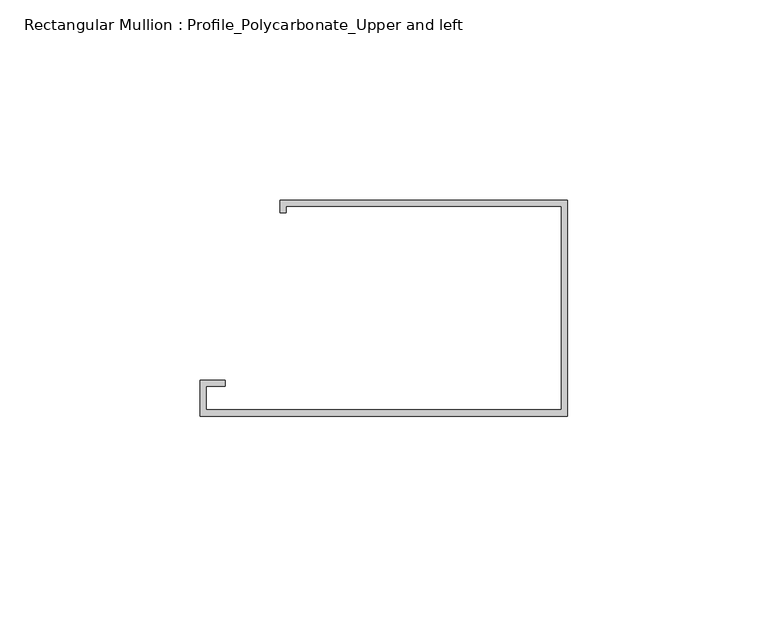
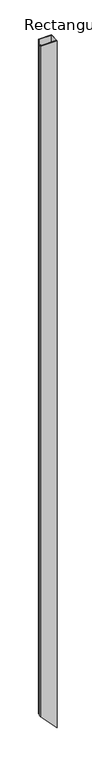
"""IFC4 building model written with IfcOpenShell, lengths in millimetres: member geometry, Rectangular Mullion : Profile_Polycarbonate_Upper and left."""

from ifc_helpers import new_model, si_unit, origin, place, context, project, spatial, faceted_brep, source, transform, mapped, element, save


def rectangular_mullion_profile_polycarbonate_upper_and_left_a20b3aa8(model_context):
    return source(origin(), model_context, "Body", "Brep", [
        faceted_brep([(0.0, -28.984575, 0.0), (0.0, 25.015825, 0.0), (-71.9836, 25.015825, 0.0), (-71.9836, 21.840825, 0.0), (-70.3961, 21.840825, 0.0), (-70.3961, 23.428325, 0.0), (-1.5875, 23.428325, 0.0), (-1.5875, -27.397075, 0.0), (-90.4113, -27.397075, 0.0), (-90.4113, -21.580475, 0.0), (-85.6488, -21.580475, 0.0), (-85.6488, -19.992975, 0.0), (-91.9988, -19.992975, 0.0), (-91.9988, -28.984575, 0.0), (0.0, -28.984575, -3990.7986929), (0.0, 25.015825, -3990.7986929), (-71.9836, 25.015825, -3915.7533176), (-71.9836, 21.840825, -3915.7533176), (-70.3961, 21.840825, -3917.4083408), (-70.3961, 23.428325, -3917.4083408), (-1.5875, 23.428325, -3989.1436696), (-1.5875, -27.397075, -3989.1436696), (-90.4113, -27.397075, -3896.5418074), (-90.4113, -21.580475, -3896.5418074), (-85.6488, -21.580475, -3901.5068772), (-85.6488, -19.992975, -3901.5068772), (-91.9988, -19.992975, -3894.8867841), (-91.9988, -28.984575, -3894.8867841)], [[[0, 1, 2, 3, 4, 5, 6, 7, 8, 9, 10, 11, 12, 13]], [[1, 0, 14, 15]], [[2, 1, 15, 16]], [[3, 2, 16, 17]], [[4, 3, 17, 18]], [[5, 4, 18, 19]], [[6, 5, 19, 20]], [[7, 6, 20, 21]], [[8, 7, 21, 22]], [[9, 8, 22, 23]], [[10, 9, 23, 24]], [[11, 10, 24, 25]], [[12, 11, 25, 26]], [[13, 12, 26, 27]], [[0, 13, 27, 14]], [[14, 27, 26, 25, 24, 23, 22, 21, 20, 19, 18, 17, 16, 15]]]),
    ])


if __name__ == "__main__":
    model = new_model("IFC4")
    model_context = context("Model", 3, world=origin())
    ifc_project = project(units=[si_unit("LENGTHUNIT", "METRE", prefix="MILLI")], contexts=[model_context])
    site = spatial("IfcSite", under=ifc_project)
    building = spatial("IfcBuilding", under=site)
    placement = place(None, origin())
    rectangular_mullion_profile_polycarbonate_upper_and_left_shape = rectangular_mullion_profile_polycarbonate_upper_and_left_a20b3aa8(model_context)
    element("IfcMember", 1, ObjectType="Rectangular Mullion : Profile_Polycarbonate_Upper and left", at=placement, inside=building, context=model_context, shape_type="MappedRepresentation", body=[
        mapped(rectangular_mullion_profile_polycarbonate_upper_and_left_shape, transform((0.0, 0.0, 0.0), x_axis=(1.0, 0.0, 0.0), y_axis=(0.0, 1.0, 0.0), z_axis=(0.0, 0.0, 1.0))),
    ])
    save(model, "model.ifc")

# Revit data of these elements
# Type "Rectangular Mullion : Profile_Polycarbonate_Upper and left"
#   built-in parameter 1007322 = 0.177167 (stored number, unit not read)
#   built-in parameter 1007321 = 0.00520833 (stored number, unit not read)
#   built-in parameter 1007320 = 0 (stored number, unit not read)
